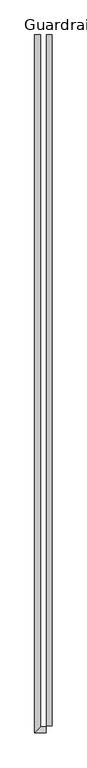
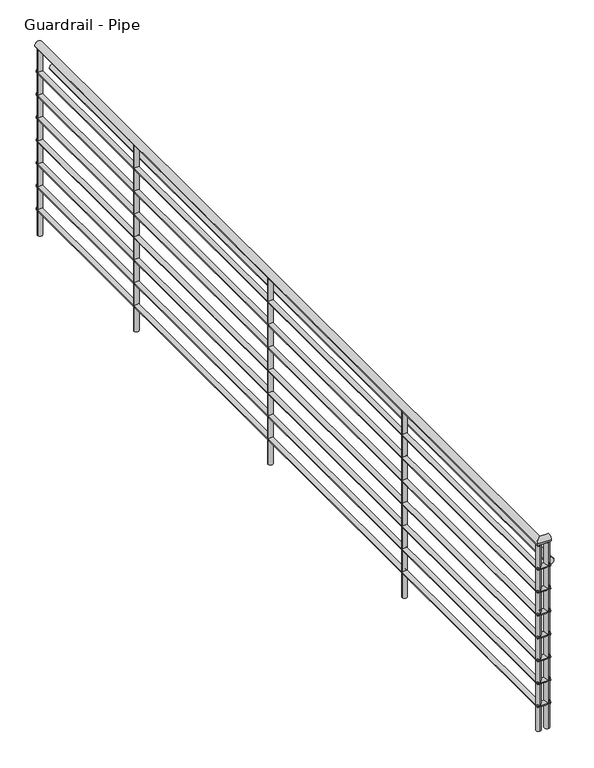
"""IFC4 building model written with IfcOpenShell, lengths in millimetres: railing geometry, Guardrail - Pipe."""

import ifcopenshell
import ifcopenshell.guid

model = None  # the IFC model being written
_history = None  # IfcOwnerHistory: only IFC2X3 demands one
_inside = {}  # id of a spatial element -> (the spatial element, [elements in it])
_under = {}  # id of a project, library or spatial element -> (it, [spatial elements below it])
_declared = {}  # id of a project -> (the project, [libraries it declares])
_typed = {}  # id of a type object -> (the type object, [elements of that type])
_made_of = {}  # id of a material, layer set ... -> (it, [elements and type objects made of it])


def new_model(schema):
    """Start an empty IFC model of exactly this schema.

    Asked for "IFC4X3", IfcOpenShell would pick the latest addendum, in which some entities
    have other attributes; the version numbers below select the first issue.
    IFC2X3 requires an IfcOwnerHistory on every rooted entity: one is made here for all.
    """
    global model, _history
    if schema == "IFC4X3":
        model = ifcopenshell.file(schema_version=(4, 3, 0, 0))
    else:
        model = ifcopenshell.file(schema=schema)
    _inside.clear()
    _under.clear()
    _declared.clear()
    _typed.clear()
    _made_of.clear()
    _history = None
    if model.schema == "IFC2X3":
        org = make("IfcOrganization", Name="unknown")
        user = make(
            "IfcPersonAndOrganization",
            ThePerson=make("IfcPerson", FamilyName="unknown"),
            TheOrganization=org,
        )
        app = make(
            "IfcApplication",
            ApplicationDeveloper=org,
            Version="unknown",
            ApplicationFullName="unknown",
            ApplicationIdentifier="unknown",
        )
        _history = make(
            "IfcOwnerHistory",
            OwningUser=user,
            OwningApplication=app,
            ChangeAction="ADDED",
            CreationDate=0,
        )
    return model


def make(cls, **values):
    """One entity of the class cls with the attributes given. An attribute that is None is left unset."""
    return model.create_entity(
        cls, **{name: value for name, value in values.items() if value is not None}
    )


def rooted(cls, **values):
    """An entity with a GlobalId (a new one), such as an element, a storey or a relation."""
    return make(cls, GlobalId=ifcopenshell.guid.new(), OwnerHistory=_history, **values)


def si_unit(unit_type, name, prefix=None):
    """IfcSIUnit, for example si_unit("LENGTHUNIT", "METRE", prefix="MILLI")."""
    return make("IfcSIUnit", UnitType=unit_type, Prefix=prefix, Name=name)


def assignment(units):
    """IfcUnitAssignment: the units of a project."""
    return None if units is None else make("IfcUnitAssignment", Units=units)


def point(xyz):
    """IfcCartesianPoint."""
    return None if xyz is None else make("IfcCartesianPoint", Coordinates=xyz)


def direction(xyz):
    """IfcDirection."""
    return None if xyz is None else make("IfcDirection", DirectionRatios=xyz)


def frame(location, z_axis=None, x_axis=None):
    """IfcAxis2Placement3D, a coordinate frame: its origin and axes. An axis left out is left unset."""
    return make(
        "IfcAxis2Placement3D",
        Location=point(location),
        Axis=direction(z_axis),
        RefDirection=direction(x_axis),
    )


def frame_2d(location, x_axis=None):
    """IfcAxis2Placement2D, a coordinate frame in the plane: its origin and x axis."""
    return make(
        "IfcAxis2Placement2D", Location=point(location), RefDirection=direction(x_axis)
    )


def origin():
    """The frame at (0, 0, 0) with its axes left unset."""
    return frame((0.0, 0.0, 0.0))


def place(relative_to, where):
    """IfcLocalPlacement: puts the frame where relative to a parent placement (None: the world)."""
    return make(
        "IfcLocalPlacement", PlacementRelTo=relative_to, RelativePlacement=where
    )


def context(
    kind, dimensions, precision=None, world=None, true_north=None, identifier=None
):
    """IfcGeometricRepresentationContext, for example the 3D "Model" context."""
    return make(
        "IfcGeometricRepresentationContext",
        ContextIdentifier=identifier,
        ContextType=kind,
        CoordinateSpaceDimension=dimensions,
        Precision=precision,
        WorldCoordinateSystem=world,
        TrueNorth=true_north,
    )


def project(units=None, contexts=None):
    """IfcProject with its units and contexts."""
    return rooted(
        "IfcProject",
        Name="project",
        RepresentationContexts=contexts,
        UnitsInContext=assignment(units),
    )


def spatial(cls, under=None, at=None, **own):
    """A site, building, storey or space (cls), placed at a placement, below another one or the project."""
    s = rooted(cls, ObjectPlacement=at, **own)
    if under is not None:
        _under.setdefault(under.id(), (under, []))[1].append(s)
    return s


def circle_curve(where, radius):
    """IfcCircle in the frame where."""
    return make("IfcCircle", Position=where, Radius=radius)


def ellipse_curve(where, semi_axis1, semi_axis2):
    """IfcEllipse in the frame where."""
    return make(
        "IfcEllipse", Position=where, SemiAxis1=semi_axis1, SemiAxis2=semi_axis2
    )


def trimmed(basis, trim1, trim2, sense, master):
    """IfcTrimmedCurve: the piece of a basis curve between two trims."""
    return make(
        "IfcTrimmedCurve",
        BasisCurve=basis,
        Trim1=trim1,
        Trim2=trim2,
        SenseAgreement=sense,
        MasterRepresentation=master,
    )


def segment(curve, same_sense, transition):
    """IfcCompositeCurveSegment."""
    return make(
        "IfcCompositeCurveSegment",
        Transition=transition,
        SameSense=same_sense,
        ParentCurve=curve,
    )


def composite_curve(segments, self_intersect=None):
    """IfcCompositeCurve: segments joined end to end."""
    return make("IfcCompositeCurve", Segments=segments, SelfIntersect=self_intersect)


def outline(outer, holes=None, kind="AREA"):
    """IfcArbitraryClosedProfileDef: a profile drawn as a closed curve; with holes, ...WithVoids."""
    if holes is None:
        return make("IfcArbitraryClosedProfileDef", ProfileType=kind, OuterCurve=outer)
    return make(
        "IfcArbitraryProfileDefWithVoids",
        ProfileType=kind,
        OuterCurve=outer,
        InnerCurves=holes,
    )


def extrude(swept, where, along, depth):
    """IfcExtrudedAreaSolid: the profile swept, set in the frame where, extruded along a direction by depth."""
    return make(
        "IfcExtrudedAreaSolid",
        SweptArea=swept,
        Position=where,
        ExtrudedDirection=direction(along),
        Depth=depth,
    )


def shape(context_of_items, identifier, shape_type, items):
    """IfcShapeRepresentation: the items that make up one representation, for example the "Body"."""
    return make(
        "IfcShapeRepresentation",
        ContextOfItems=context_of_items,
        RepresentationIdentifier=identifier,
        RepresentationType=shape_type,
        Items=items,
    )


def source(mapping_origin, context_of_items, identifier, shape_type, items):
    """IfcRepresentationMap: a shape defined once, which mapped items show again and again."""
    return make(
        "IfcRepresentationMap",
        MappingOrigin=mapping_origin,
        MappedRepresentation=shape(context_of_items, identifier, shape_type, items),
    )


def transform(
    local_origin,
    x_axis=None,
    y_axis=None,
    z_axis=None,
    scale=None,
    scale2=None,
    scale3=None,
    uniform=True,
):
    """IfcCartesianTransformationOperator3D, or its non-uniform kind. x_axis, y_axis, z_axis: its Axis1, 2, 3."""
    if uniform:
        return make(
            "IfcCartesianTransformationOperator3D",
            Axis1=direction(x_axis),
            Axis2=direction(y_axis),
            LocalOrigin=point(local_origin),
            Scale=scale,
            Axis3=direction(z_axis),
        )
    return make(
        "IfcCartesianTransformationOperator3DnonUniform",
        Axis1=direction(x_axis),
        Axis2=direction(y_axis),
        LocalOrigin=point(local_origin),
        Scale=scale,
        Axis3=direction(z_axis),
        Scale2=scale2,
        Scale3=scale3,
    )


def mapped(mapping_source, mapping_target):
    """IfcMappedItem: shows the shape of a source again, moved by a transform."""
    return make(
        "IfcMappedItem", MappingSource=mapping_source, MappingTarget=mapping_target
    )


def made_of(thing, what):
    """Note that an element or type object is made of a material, layer set ...; save() writes the relation."""
    if what is not None:
        _made_of.setdefault(what.id(), (what, []))[1].append(thing)
    return thing


def element(
    cls,
    number,
    at=None,
    inside=None,
    cuts=None,
    type_object=None,
    material=None,
    context=None,
    identifier="Body",
    shape_type=None,
    held_by="IfcProductDefinitionShape",
    body=None,
    shapes=None,
    **own,
):
    """One element of the class cls, such as IfcWall. Its Tag is "e" and its number.

    at: its placement. inside: the storey or other place that contains it. cuts: it is an
    opening in that element (IfcRelVoidsElement). A single representation is given by context,
    identifier, shape_type and body (its items); several are given by shapes. held_by: the class
    of the entity that holds the representations. save() writes the other relations.
    """
    e = rooted(cls, Tag="e%d" % number, ObjectPlacement=at, **own)
    if body is not None:
        shapes = [shape(context, identifier, shape_type, body)]
    if shapes is not None:
        e.Representation = make(held_by, Representations=shapes)
    if inside is not None:
        _inside.setdefault(inside.id(), (inside, []))[1].append(e)
    if cuts is not None:
        rooted(
            "IfcRelVoidsElement", RelatingBuildingElement=cuts, RelatedOpeningElement=e
        )
    if type_object is not None:
        _typed.setdefault(type_object.id(), (type_object, []))[1].append(e)
    return made_of(e, material)


def aggregate(whole, parts):
    """IfcRelAggregates: a whole, such as a stair, and the parts it consists of."""
    return rooted("IfcRelAggregates", RelatingObject=whole, RelatedObjects=parts)


def save(model, path):
    """Write the relations noted so far, then the file.

    IfcRelAggregates (storeys below a building ...), IfcRelContainedInSpatialStructure (elements
    in a storey), IfcRelDefinesByType, IfcRelAssociatesMaterial and IfcRelDeclares: one each for
    every whole, place, type object, material and project.
    """
    for whole, parts in _under.values():
        aggregate(whole, parts)
    for where, things in _inside.values():
        rooted(
            "IfcRelContainedInSpatialStructure",
            RelatedElements=things,
            RelatingStructure=where,
        )
    for kind, things in _typed.values():
        rooted("IfcRelDefinesByType", RelatedObjects=things, RelatingType=kind)
    for what, things in _made_of.values():
        rooted("IfcRelAssociatesMaterial", RelatedObjects=things, RelatingMaterial=what)
    for by, libraries in _declared.values():
        rooted("IfcRelDeclares", RelatingContext=by, RelatedDefinitions=libraries)
    model.write(path)


def plane_surface(at):
    """IfcPlane: the flat surface through the origin of the frame at, square to its z axis."""
    return make("IfcPlane", Position=at)


def cylinder_surface(at, radius):
    """IfcCylindricalSurface: all points at the distance radius from the z axis of the frame at."""
    return make("IfcCylindricalSurface", Position=at, Radius=radius)


def advanced_brep(points, edges, surfaces, faces):
    """IfcAdvancedBrep: a solid bounded by faces that lie on surfaces and meet in shared edges.

    An edge is (start, end): straight between two places in points (the first is 0);
    or (start, end, curve); or (start, end, curve, False) where it runs against its curve.
    A face is (place in surfaces, loops), or (place, loops, False) where it looks against
    its surface's normal. A loop lists edges by number (the first is 1), with a minus sign
    where the edge is run from its end to its start. The first loop is the outer one.
    """
    corners = [point(p) for p in points]
    vertices = [make("IfcVertexPoint", VertexGeometry=c) for c in corners]
    made = []
    for start, end, *more in edges:
        made.append(
            make(
                "IfcEdgeCurve",
                EdgeStart=vertices[start],
                EdgeEnd=vertices[end],
                EdgeGeometry=more[0] if more else make("IfcPolyline", Points=[corners[start], corners[end]]),
                SameSense=more[1] if len(more) > 1 else True,
            )
        )
    hull = []
    for where, loops, *sense in faces:
        bounds = []
        for j, loop in enumerate(loops):
            ring = [make("IfcOrientedEdge", EdgeElement=made[abs(k) - 1], Orientation=k > 0) for k in loop]
            bounds.append(
                make(
                    "IfcFaceOuterBound" if j == 0 else "IfcFaceBound",
                    Bound=make("IfcEdgeLoop", EdgeList=ring),
                    Orientation=True,
                )
            )
        hull.append(make("IfcAdvancedFace", Bounds=bounds, FaceSurface=surfaces[where], SameSense=sense[0] if sense else True))
    return make("IfcAdvancedBrep", Outer=make("IfcClosedShell", CfsFaces=hull))


def guardrail_pipe_4d6737b3(model_context):
    return source(origin(), model_context, "Body", "SolidModel", [
        advanced_brep(
        [(-10682.1293787, 596.0663228, 4705.35), (-10720.2293787, 596.0663228, 4705.35), (-10682.1293787, -3931.4836772, 4705.35), (-10720.2293787, -3969.5836772, 4705.35), (-10645.1029016, -3931.4836772, 4705.35), (-10645.1029016, -3969.5836772, 4705.35)],
        [
            (0, 1, circle_curve(frame((-10701.1793787, 596.0663228, 4705.35), z_axis=(0.0, 1.0, 0.0), x_axis=(-1.0, 0.0, 0.0)), 19.05)),
            (1, 0, circle_curve(frame((-10701.1793787, 596.0663228, 4705.35), z_axis=(0.0, 1.0, 0.0), x_axis=(-1.0, 0.0, 0.0)), 19.05)),
            (2, 3, ellipse_curve(frame((-10701.1793787, -3950.5336772, 4705.35), z_axis=(-0.7071067811865456, 0.7071067811865493, 0.0), x_axis=(-0.7071067811865492, -0.7071067811865458, 0.0)), 26.9407684, 19.05)),
            (3, 1),
            (0, 2),
            (3, 2, ellipse_curve(frame((-10701.1793787, -3950.5336772, 4705.35), z_axis=(-0.7071067811865456, 0.7071067811865493, 0.0), x_axis=(-0.7071067811865492, -0.7071067811865458, 0.0)), 26.9407684, 19.05)),
            (4, 5, circle_curve(frame((-10645.1029016, -3950.5336772, 4705.35), z_axis=(1.0, 0.0, 0.0), x_axis=(0.0, -1.0, 0.0)), 19.05)),
            (5, 4, circle_curve(frame((-10645.1029016, -3950.5336772, 4705.35), z_axis=(1.0, 0.0, 0.0), x_axis=(0.0, -1.0, 0.0)), 19.05)),
            (5, 3),
            (2, 4),
        ],
        [
            plane_surface(frame((-10701.1793787, 596.0663228, 4724.4), z_axis=(0.0, 1.0, 0.0), x_axis=(0.0, 0.0, 1.0))),
            cylinder_surface(frame((-10701.1793787, -3950.5336772, 4705.35), z_axis=(0.0, -1.0, 0.0), x_axis=(-1.0, 0.0, 0.0)), 19.05),
            plane_surface(frame((-10645.1029016, -3950.5336772, 4724.4), z_axis=(1.0, 0.0, 0.0), x_axis=(0.0, -1.0, 0.0))),
            cylinder_surface(frame((-10645.1029016, -3950.5336772, 4705.35), z_axis=(1.0, 0.0, 0.0), x_axis=(0.0, -1.0, 0.0)), 19.05),
        ],
        [
            (0, [[1, 2]]),
            (1, [[3, 4, -1, 5]]),
            (1, [[6, -5, -2, -4]]),
            (2, [[7, 8]]),
            (3, [[-8, 9, -3, 10]]),
            (3, [[-7, -10, -6, -9]]),
        ],
    ),
        advanced_brep(
        [(-10688.4793787, 596.0663228, 4559.3), (-10713.8793787, 596.0663228, 4559.3), (-10688.4793787, -3937.8336772, 4559.3), (-10713.8793787, -3963.2336772, 4559.3), (-10645.1029016, -3937.8336772, 4559.3), (-10645.1029016, -3963.2336772, 4559.3)],
        [
            (0, 1, circle_curve(frame((-10701.1793787, 596.0663228, 4559.3), z_axis=(0.0, 1.0, 0.0), x_axis=(-1.0, 0.0, 0.0)), 12.7)),
            (1, 0, circle_curve(frame((-10701.1793787, 596.0663228, 4559.3), z_axis=(0.0, 1.0, 0.0), x_axis=(-1.0, 0.0, 0.0)), 12.7)),
            (2, 3, ellipse_curve(frame((-10701.1793787, -3950.5336772, 4559.3), z_axis=(-0.7071067811865456, 0.7071067811865493, 0.0), x_axis=(-0.7071067811865492, -0.7071067811865458, 0.0)), 17.9605122, 12.7)),
            (3, 1),
            (0, 2),
            (3, 2, ellipse_curve(frame((-10701.1793787, -3950.5336772, 4559.3), z_axis=(-0.7071067811865456, 0.7071067811865493, 0.0), x_axis=(-0.7071067811865492, -0.7071067811865458, 0.0)), 17.9605122, 12.7)),
            (4, 5, circle_curve(frame((-10645.1029016, -3950.5336772, 4559.3), z_axis=(1.0, 0.0, 0.0), x_axis=(0.0, -1.0, 0.0)), 12.7)),
            (5, 4, circle_curve(frame((-10645.1029016, -3950.5336772, 4559.3), z_axis=(1.0, 0.0, 0.0), x_axis=(0.0, -1.0, 0.0)), 12.7)),
            (4, 2),
            (3, 5),
        ],
        [
            plane_surface(frame((-10701.1793787, 596.0663228, 4572.0), z_axis=(0.0, 1.0, 0.0), x_axis=(0.0, 0.0, 1.0))),
            cylinder_surface(frame((-10701.1793787, -3950.5336772, 4559.3), z_axis=(0.0, -1.0, 0.0), x_axis=(-1.0, 0.0, 0.0)), 12.7),
            plane_surface(frame((-10645.1029016, -3950.5336772, 4572.0), z_axis=(1.0, 0.0, 0.0), x_axis=(0.0, -1.0, 0.0))),
            cylinder_surface(frame((-10645.1029016, -3950.5336772, 4559.3), z_axis=(1.0, 0.0, 0.0), x_axis=(0.0, -1.0, 0.0)), 12.7),
        ],
        [
            (0, [[1, 2]]),
            (1, [[3, 4, -1, 5]]),
            (1, [[6, -5, -2, -4]]),
            (2, [[7, 8]]),
            (3, [[-7, 9, -6, 10]]),
            (3, [[-8, -10, -3, -9]]),
        ],
    ),
        advanced_brep(
        [(-10605.9293787, -3925.1336772, 4552.95), (-10644.0293787, -3925.1336772, 4552.95), (-10605.9293787, 596.0663228, 4552.95), (-10644.0293787, 596.0663228, 4552.95)],
        [
            (0, 1, circle_curve(frame((-10624.9793787, -3925.1336772, 4552.95), z_axis=(0.0, -1.0, 0.0), x_axis=(-1.0, 0.0, 0.0)), 19.05)),
            (1, 0, circle_curve(frame((-10624.9793787, -3925.1336772, 4552.95), z_axis=(0.0, -1.0, 0.0), x_axis=(-1.0, 0.0, 0.0)), 19.05)),
            (2, 3, circle_curve(frame((-10624.9793787, 596.0663228, 4552.95), z_axis=(0.0, 1.0, 0.0), x_axis=(-1.0, 0.0, 0.0)), 19.05)),
            (3, 2, circle_curve(frame((-10624.9793787, 596.0663228, 4552.95), z_axis=(0.0, 1.0, 0.0), x_axis=(-1.0, 0.0, 0.0)), 19.05)),
            (1, 3),
            (2, 0),
        ],
        [
            plane_surface(frame((-10624.9793787, -3925.1336772, 4572.0), z_axis=(0.0, -1.0, 0.0), x_axis=(0.0, 0.0, 1.0))),
            plane_surface(frame((-10624.9793787, 596.0663228, 4572.0), z_axis=(0.0, 1.0, 0.0), x_axis=(0.0, 0.0, 1.0))),
            cylinder_surface(frame((-10624.9793787, -3925.1336772, 4552.95), z_axis=(0.0, -1.0, 0.0), x_axis=(-1.0, 0.0, 0.0)), 19.05),
        ],
        [
            (0, [[1, 2]]),
            (1, [[3, 4]]),
            (2, [[-2, 5, -3, 6]]),
            (2, [[-1, -6, -4, -5]]),
        ],
    ),
        advanced_brep(
        [(-10688.4793787, 596.0663228, 4432.3), (-10713.8793787, 596.0663228, 4432.3), (-10688.4793787, -3937.8336772, 4432.3), (-10713.8793787, -3963.2336772, 4432.3), (-10645.1029016, -3937.8336772, 4432.3), (-10645.1029016, -3963.2336772, 4432.3)],
        [
            (0, 1, circle_curve(frame((-10701.1793787, 596.0663228, 4432.3), z_axis=(0.0, 1.0, 0.0), x_axis=(-1.0, 0.0, 0.0)), 12.7)),
            (1, 0, circle_curve(frame((-10701.1793787, 596.0663228, 4432.3), z_axis=(0.0, 1.0, 0.0), x_axis=(-1.0, 0.0, 0.0)), 12.7)),
            (2, 3, ellipse_curve(frame((-10701.1793787, -3950.5336772, 4432.3), z_axis=(-0.7071067811865456, 0.7071067811865493, 0.0), x_axis=(-0.7071067811865492, -0.7071067811865458, 0.0)), 17.9605122, 12.7)),
            (3, 1),
            (0, 2),
            (3, 2, ellipse_curve(frame((-10701.1793787, -3950.5336772, 4432.3), z_axis=(-0.7071067811865456, 0.7071067811865493, 0.0), x_axis=(-0.7071067811865492, -0.7071067811865458, 0.0)), 17.9605122, 12.7)),
            (4, 5, circle_curve(frame((-10645.1029016, -3950.5336772, 4432.3), z_axis=(1.0, 0.0, 0.0), x_axis=(0.0, -1.0, 0.0)), 12.7)),
            (5, 4, circle_curve(frame((-10645.1029016, -3950.5336772, 4432.3), z_axis=(1.0, 0.0, 0.0), x_axis=(0.0, -1.0, 0.0)), 12.7)),
            (4, 2),
            (3, 5),
        ],
        [
            plane_surface(frame((-10701.1793787, 596.0663228, 4445.0), z_axis=(0.0, 1.0, 0.0), x_axis=(0.0, 0.0, 1.0))),
            cylinder_surface(frame((-10701.1793787, -3950.5336772, 4432.3), z_axis=(0.0, -1.0, 0.0), x_axis=(-1.0, 0.0, 0.0)), 12.7),
            plane_surface(frame((-10645.1029016, -3950.5336772, 4445.0), z_axis=(1.0, 0.0, 0.0), x_axis=(0.0, -1.0, 0.0))),
            cylinder_surface(frame((-10645.1029016, -3950.5336772, 4432.3), z_axis=(1.0, 0.0, 0.0), x_axis=(0.0, -1.0, 0.0)), 12.7),
        ],
        [
            (0, [[1, 2]]),
            (1, [[3, 4, -1, 5]]),
            (1, [[6, -5, -2, -4]]),
            (2, [[7, 8]]),
            (3, [[-7, 9, -6, 10]]),
            (3, [[-8, -10, -3, -9]]),
        ],
    ),
        advanced_brep(
        [(-10688.4793787, 596.0663228, 4305.3), (-10713.8793787, 596.0663228, 4305.3), (-10688.4793787, -3937.8336772, 4305.3), (-10713.8793787, -3963.2336772, 4305.3), (-10645.1029016, -3937.8336772, 4305.3), (-10645.1029016, -3963.2336772, 4305.3)],
        [
            (0, 1, circle_curve(frame((-10701.1793787, 596.0663228, 4305.3), z_axis=(0.0, 1.0, 0.0), x_axis=(-1.0, 0.0, 0.0)), 12.7)),
            (1, 0, circle_curve(frame((-10701.1793787, 596.0663228, 4305.3), z_axis=(0.0, 1.0, 0.0), x_axis=(-1.0, 0.0, 0.0)), 12.7)),
            (2, 3, ellipse_curve(frame((-10701.1793787, -3950.5336772, 4305.3), z_axis=(-0.7071067811865456, 0.7071067811865493, 0.0), x_axis=(-0.7071067811865492, -0.7071067811865458, 0.0)), 17.9605122, 12.7)),
            (3, 1),
            (0, 2),
            (3, 2, ellipse_curve(frame((-10701.1793787, -3950.5336772, 4305.3), z_axis=(-0.7071067811865456, 0.7071067811865493, 0.0), x_axis=(-0.7071067811865492, -0.7071067811865458, 0.0)), 17.9605122, 12.7)),
            (4, 5, circle_curve(frame((-10645.1029016, -3950.5336772, 4305.3), z_axis=(1.0, 0.0, 0.0), x_axis=(0.0, -1.0, 0.0)), 12.7)),
            (5, 4, circle_curve(frame((-10645.1029016, -3950.5336772, 4305.3), z_axis=(1.0, 0.0, 0.0), x_axis=(0.0, -1.0, 0.0)), 12.7)),
            (4, 2),
            (3, 5),
        ],
        [
            plane_surface(frame((-10701.1793787, 596.0663228, 4318.0), z_axis=(0.0, 1.0, 0.0), x_axis=(0.0, 0.0, 1.0))),
            cylinder_surface(frame((-10701.1793787, -3950.5336772, 4305.3), z_axis=(0.0, -1.0, 0.0), x_axis=(-1.0, 0.0, 0.0)), 12.7),
            plane_surface(frame((-10645.1029016, -3950.5336772, 4318.0), z_axis=(1.0, 0.0, 0.0), x_axis=(0.0, -1.0, 0.0))),
            cylinder_surface(frame((-10645.1029016, -3950.5336772, 4305.3), z_axis=(1.0, 0.0, 0.0), x_axis=(0.0, -1.0, 0.0)), 12.7),
        ],
        [
            (0, [[1, 2]]),
            (1, [[3, 4, -1, 5]]),
            (1, [[6, -5, -2, -4]]),
            (2, [[7, 8]]),
            (3, [[-7, 9, -6, 10]]),
            (3, [[-8, -10, -3, -9]]),
        ],
    ),
        advanced_brep(
        [(-10688.4793787, 596.0663228, 4178.3), (-10713.8793787, 596.0663228, 4178.3), (-10688.4793787, -3937.8336772, 4178.3), (-10713.8793787, -3963.2336772, 4178.3), (-10645.1029016, -3937.8336772, 4178.3), (-10645.1029016, -3963.2336772, 4178.3)],
        [
            (0, 1, circle_curve(frame((-10701.1793787, 596.0663228, 4178.3), z_axis=(0.0, 1.0, 0.0), x_axis=(-1.0, 0.0, 0.0)), 12.7)),
            (1, 0, circle_curve(frame((-10701.1793787, 596.0663228, 4178.3), z_axis=(0.0, 1.0, 0.0), x_axis=(-1.0, 0.0, 0.0)), 12.7)),
            (2, 3, ellipse_curve(frame((-10701.1793787, -3950.5336772, 4178.3), z_axis=(-0.7071067811865456, 0.7071067811865493, 0.0), x_axis=(-0.7071067811865492, -0.7071067811865458, 0.0)), 17.9605122, 12.7)),
            (3, 1),
            (0, 2),
            (3, 2, ellipse_curve(frame((-10701.1793787, -3950.5336772, 4178.3), z_axis=(-0.7071067811865456, 0.7071067811865493, 0.0), x_axis=(-0.7071067811865492, -0.7071067811865458, 0.0)), 17.9605122, 12.7)),
            (4, 5, circle_curve(frame((-10645.1029016, -3950.5336772, 4178.3), z_axis=(1.0, 0.0, 0.0), x_axis=(0.0, -1.0, 0.0)), 12.7)),
            (5, 4, circle_curve(frame((-10645.1029016, -3950.5336772, 4178.3), z_axis=(1.0, 0.0, 0.0), x_axis=(0.0, -1.0, 0.0)), 12.7)),
            (4, 2),
            (3, 5),
        ],
        [
            plane_surface(frame((-10701.1793787, 596.0663228, 4191.0), z_axis=(0.0, 1.0, 0.0), x_axis=(0.0, 0.0, 1.0))),
            cylinder_surface(frame((-10701.1793787, -3950.5336772, 4178.3), z_axis=(0.0, -1.0, 0.0), x_axis=(-1.0, 0.0, 0.0)), 12.7),
            plane_surface(frame((-10645.1029016, -3950.5336772, 4191.0), z_axis=(1.0, 0.0, 0.0), x_axis=(0.0, -1.0, 0.0))),
            cylinder_surface(frame((-10645.1029016, -3950.5336772, 4178.3), z_axis=(1.0, 0.0, 0.0), x_axis=(0.0, -1.0, 0.0)), 12.7),
        ],
        [
            (0, [[1, 2]]),
            (1, [[3, 4, -1, 5]]),
            (1, [[6, -5, -2, -4]]),
            (2, [[7, 8]]),
            (3, [[-7, 9, -6, 10]]),
            (3, [[-8, -10, -3, -9]]),
        ],
    ),
        advanced_brep(
        [(-10688.4793787, 596.0663228, 4051.3), (-10713.8793787, 596.0663228, 4051.3), (-10688.4793787, -3937.8336772, 4051.3), (-10713.8793787, -3963.2336772, 4051.3), (-10645.1029016, -3937.8336772, 4051.3), (-10645.1029016, -3963.2336772, 4051.3)],
        [
            (0, 1, circle_curve(frame((-10701.1793787, 596.0663228, 4051.3), z_axis=(0.0, 1.0, 0.0), x_axis=(-1.0, 0.0, 0.0)), 12.7)),
            (1, 0, circle_curve(frame((-10701.1793787, 596.0663228, 4051.3), z_axis=(0.0, 1.0, 0.0), x_axis=(-1.0, 0.0, 0.0)), 12.7)),
            (2, 3, ellipse_curve(frame((-10701.1793787, -3950.5336772, 4051.3), z_axis=(-0.7071067811865456, 0.7071067811865493, 0.0), x_axis=(-0.7071067811865492, -0.7071067811865458, 0.0)), 17.9605122, 12.7)),
            (3, 1),
            (0, 2),
            (3, 2, ellipse_curve(frame((-10701.1793787, -3950.5336772, 4051.3), z_axis=(-0.7071067811865456, 0.7071067811865493, 0.0), x_axis=(-0.7071067811865492, -0.7071067811865458, 0.0)), 17.9605122, 12.7)),
            (4, 5, circle_curve(frame((-10645.1029016, -3950.5336772, 4051.3), z_axis=(1.0, 0.0, 0.0), x_axis=(0.0, -1.0, 0.0)), 12.7)),
            (5, 4, circle_curve(frame((-10645.1029016, -3950.5336772, 4051.3), z_axis=(1.0, 0.0, 0.0), x_axis=(0.0, -1.0, 0.0)), 12.7)),
            (4, 2),
            (3, 5),
        ],
        [
            plane_surface(frame((-10701.1793787, 596.0663228, 4064.0), z_axis=(0.0, 1.0, 0.0), x_axis=(0.0, 0.0, 1.0))),
            cylinder_surface(frame((-10701.1793787, -3950.5336772, 4051.3), z_axis=(0.0, -1.0, 0.0), x_axis=(-1.0, 0.0, 0.0)), 12.7),
            plane_surface(frame((-10645.1029016, -3950.5336772, 4064.0), z_axis=(1.0, 0.0, 0.0), x_axis=(0.0, -1.0, 0.0))),
            cylinder_surface(frame((-10645.1029016, -3950.5336772, 4051.3), z_axis=(1.0, 0.0, 0.0), x_axis=(0.0, -1.0, 0.0)), 12.7),
        ],
        [
            (0, [[1, 2]]),
            (1, [[3, 4, -1, 5]]),
            (1, [[6, -5, -2, -4]]),
            (2, [[7, 8]]),
            (3, [[-7, 9, -6, 10]]),
            (3, [[-8, -10, -3, -9]]),
        ],
    ),
        advanced_brep(
        [(-10688.4793787, 596.0663228, 3924.3), (-10713.8793787, 596.0663228, 3924.3), (-10688.4793787, -3937.8336772, 3924.3), (-10713.8793787, -3963.2336772, 3924.3), (-10645.1029016, -3937.8336772, 3924.3), (-10645.1029016, -3963.2336772, 3924.3)],
        [
            (0, 1, circle_curve(frame((-10701.1793787, 596.0663228, 3924.3), z_axis=(0.0, 1.0, 0.0), x_axis=(-1.0, 0.0, 0.0)), 12.7)),
            (1, 0, circle_curve(frame((-10701.1793787, 596.0663228, 3924.3), z_axis=(0.0, 1.0, 0.0), x_axis=(-1.0, 0.0, 0.0)), 12.7)),
            (2, 3, ellipse_curve(frame((-10701.1793787, -3950.5336772, 3924.3), z_axis=(-0.7071067811865456, 0.7071067811865493, 0.0), x_axis=(-0.7071067811865492, -0.7071067811865458, 0.0)), 17.9605122, 12.7)),
            (3, 1),
            (0, 2),
            (3, 2, ellipse_curve(frame((-10701.1793787, -3950.5336772, 3924.3), z_axis=(-0.7071067811865456, 0.7071067811865493, 0.0), x_axis=(-0.7071067811865492, -0.7071067811865458, 0.0)), 17.9605122, 12.7)),
            (4, 5, circle_curve(frame((-10645.1029016, -3950.5336772, 3924.3), z_axis=(1.0, 0.0, 0.0), x_axis=(0.0, -1.0, 0.0)), 12.7)),
            (5, 4, circle_curve(frame((-10645.1029016, -3950.5336772, 3924.3), z_axis=(1.0, 0.0, 0.0), x_axis=(0.0, -1.0, 0.0)), 12.7)),
            (4, 2),
            (3, 5),
        ],
        [
            plane_surface(frame((-10701.1793787, 596.0663228, 3937.0), z_axis=(0.0, 1.0, 0.0), x_axis=(0.0, 0.0, 1.0))),
            cylinder_surface(frame((-10701.1793787, -3950.5336772, 3924.3), z_axis=(0.0, -1.0, 0.0), x_axis=(-1.0, 0.0, 0.0)), 12.7),
            plane_surface(frame((-10645.1029016, -3950.5336772, 3937.0), z_axis=(1.0, 0.0, 0.0), x_axis=(0.0, -1.0, 0.0))),
            cylinder_surface(frame((-10645.1029016, -3950.5336772, 3924.3), z_axis=(1.0, 0.0, 0.0), x_axis=(0.0, -1.0, 0.0)), 12.7),
        ],
        [
            (0, [[1, 2]]),
            (1, [[3, 4, -1, 5]]),
            (1, [[6, -5, -2, -4]]),
            (2, [[7, 8]]),
            (3, [[-7, 9, -6, 10]]),
            (3, [[-8, -10, -3, -9]]),
        ],
    ),
        advanced_brep(
        [(-10688.4793787, 596.0663228, 3797.3), (-10713.8793787, 596.0663228, 3797.3), (-10688.4793787, -3937.8336772, 3797.3), (-10713.8793787, -3963.2336772, 3797.3), (-10645.1029016, -3937.8336772, 3797.3), (-10645.1029016, -3963.2336772, 3797.3)],
        [
            (0, 1, circle_curve(frame((-10701.1793787, 596.0663228, 3797.3), z_axis=(0.0, 1.0, 0.0), x_axis=(-1.0, 0.0, 0.0)), 12.7)),
            (1, 0, circle_curve(frame((-10701.1793787, 596.0663228, 3797.3), z_axis=(0.0, 1.0, 0.0), x_axis=(-1.0, 0.0, 0.0)), 12.7)),
            (2, 3, ellipse_curve(frame((-10701.1793787, -3950.5336772, 3797.3), z_axis=(-0.7071067811865456, 0.7071067811865493, 0.0), x_axis=(-0.7071067811865492, -0.7071067811865458, 0.0)), 17.9605122, 12.7)),
            (3, 1),
            (0, 2),
            (3, 2, ellipse_curve(frame((-10701.1793787, -3950.5336772, 3797.3), z_axis=(-0.7071067811865456, 0.7071067811865493, 0.0), x_axis=(-0.7071067811865492, -0.7071067811865458, 0.0)), 17.9605122, 12.7)),
            (4, 5, circle_curve(frame((-10645.1029016, -3950.5336772, 3797.3), z_axis=(1.0, 0.0, 0.0), x_axis=(0.0, -1.0, 0.0)), 12.7)),
            (5, 4, circle_curve(frame((-10645.1029016, -3950.5336772, 3797.3), z_axis=(1.0, 0.0, 0.0), x_axis=(0.0, -1.0, 0.0)), 12.7)),
            (4, 2),
            (3, 5),
        ],
        [
            plane_surface(frame((-10701.1793787, 596.0663228, 3810.0), z_axis=(0.0, 1.0, 0.0), x_axis=(0.0, 0.0, 1.0))),
            cylinder_surface(frame((-10701.1793787, -3950.5336772, 3797.3), z_axis=(0.0, -1.0, 0.0), x_axis=(-1.0, 0.0, 0.0)), 12.7),
            plane_surface(frame((-10645.1029016, -3950.5336772, 3810.0), z_axis=(1.0, 0.0, 0.0), x_axis=(0.0, -1.0, 0.0))),
            cylinder_surface(frame((-10645.1029016, -3950.5336772, 3797.3), z_axis=(1.0, 0.0, 0.0), x_axis=(0.0, -1.0, 0.0)), 12.7),
        ],
        [
            (0, [[1, 2]]),
            (1, [[3, 4, -1, 5]]),
            (1, [[6, -5, -2, -4]]),
            (2, [[7, 8]]),
            (3, [[-7, 9, -6, 10]]),
            (3, [[-8, -10, -3, -9]]),
        ],
    ),
        extrude(outline(composite_curve([segment(trimmed(circle_curve(frame_2d((-10701.1793787, -292.9336772)), 12.7), [point((-10688.4793787, -292.9336772))], [point((-10713.8793787, -292.9336772))], False, "CARTESIAN"), True, "CONTINUOUS"), segment(trimmed(circle_curve(frame_2d((-10701.1793787, -292.9336772)), 12.7), [point((-10713.8793787, -292.9336772))], [point((-10688.4793787, -292.9336772))], False, "CARTESIAN"), True, "CONTINUOUS")], self_intersect=False)), frame((0.0, 0.0, 3657.6), z_axis=(0.0, 0.0, 1.0), x_axis=(1.0, 0.0, 0.0)), (0.0, 0.0, 1.0), 1028.7),
        extrude(outline(composite_curve([segment(trimmed(circle_curve(frame_2d((-10701.1793787, -1512.1336772)), 12.7), [point((-10688.4793787, -1512.1336772))], [point((-10713.8793787, -1512.1336772))], False, "CARTESIAN"), True, "CONTINUOUS"), segment(trimmed(circle_curve(frame_2d((-10701.1793787, -1512.1336772)), 12.7), [point((-10713.8793787, -1512.1336772))], [point((-10688.4793787, -1512.1336772))], False, "CARTESIAN"), True, "CONTINUOUS")], self_intersect=False)), frame((0.0, 0.0, 3657.6), z_axis=(0.0, 0.0, 1.0), x_axis=(1.0, 0.0, 0.0)), (0.0, 0.0, 1.0), 1028.7),
        extrude(outline(composite_curve([segment(trimmed(circle_curve(frame_2d((-10701.1793787, -2731.3336772)), 12.7), [point((-10688.4793787, -2731.3336772))], [point((-10713.8793787, -2731.3336772))], False, "CARTESIAN"), True, "CONTINUOUS"), segment(trimmed(circle_curve(frame_2d((-10701.1793787, -2731.3336772)), 12.7), [point((-10713.8793787, -2731.3336772))], [point((-10688.4793787, -2731.3336772))], False, "CARTESIAN"), True, "CONTINUOUS")], self_intersect=False)), frame((0.0, 0.0, 3657.6), z_axis=(0.0, 0.0, 1.0), x_axis=(1.0, 0.0, 0.0)), (0.0, 0.0, 1.0), 1028.7),
        extrude(outline(composite_curve([segment(trimmed(circle_curve(frame_2d((-10701.1793787, -3950.5336772)), 12.7), [point((-10701.1793787, -3937.8336772))], [point((-10701.1793787, -3963.2336772))], False, "CARTESIAN"), True, "CONTINUOUS"), segment(trimmed(circle_curve(frame_2d((-10701.1793787, -3950.5336772)), 12.7), [point((-10701.1793787, -3963.2336772))], [point((-10701.1793787, -3937.8336772))], False, "CARTESIAN"), True, "CONTINUOUS")], self_intersect=False)), frame((0.0, 0.0, 3657.6), z_axis=(0.0, 0.0, 1.0), x_axis=(1.0, 0.0, 0.0)), (0.0, 0.0, 1.0), 1028.7),
        extrude(outline(composite_curve([segment(trimmed(circle_curve(frame_2d((-10701.1793787, 583.3663228)), 12.7), [point((-10688.4793787, 583.3663228))], [point((-10713.8793787, 583.3663228))], False, "CARTESIAN"), True, "CONTINUOUS"), segment(trimmed(circle_curve(frame_2d((-10701.1793787, 583.3663228)), 12.7), [point((-10713.8793787, 583.3663228))], [point((-10688.4793787, 583.3663228))], False, "CARTESIAN"), True, "CONTINUOUS")], self_intersect=False)), frame((0.0, 0.0, 3657.6), z_axis=(0.0, 0.0, 1.0), x_axis=(1.0, 0.0, 0.0)), (0.0, 0.0, 1.0), 1028.7),
        extrude(outline(composite_curve([segment(trimmed(circle_curve(frame_2d((-10657.8029016, -3950.5336772)), 12.7), [point((-10657.8029016, -3937.8336772))], [point((-10657.8029016, -3963.2336772))], False, "CARTESIAN"), True, "CONTINUOUS"), segment(trimmed(circle_curve(frame_2d((-10657.8029016, -3950.5336772)), 12.7), [point((-10657.8029016, -3963.2336772))], [point((-10657.8029016, -3937.8336772))], False, "CARTESIAN"), True, "CONTINUOUS")], self_intersect=False)), frame((0.0, 0.0, 3657.6), z_axis=(0.0, 0.0, 1.0), x_axis=(1.0, 0.0, 0.0)), (0.0, 0.0, 1.0), 1028.7),
    ])


if __name__ == "__main__":
    model = new_model("IFC4")
    model_context = context("Model", 3, world=origin())
    ifc_project = project(units=[si_unit("LENGTHUNIT", "METRE", prefix="MILLI")], contexts=[model_context])
    site = spatial("IfcSite", under=ifc_project)
    building = spatial("IfcBuilding", under=site)
    placement = place(None, origin())
    guardrail_pipe_shape = guardrail_pipe_4d6737b3(model_context)
    element("IfcRailing", 1, ObjectType="Guardrail - Pipe", at=placement, inside=building, context=model_context, shape_type="MappedRepresentation", body=[
        mapped(guardrail_pipe_shape, transform((0.0, 0.0, 0.0), x_axis=(1.0, 0.0, 0.0), y_axis=(0.0, 1.0, 0.0), z_axis=(0.0, 0.0, 1.0))),
    ])
    save(model, "model.ifc")

# Revit data of these elements
# Element 1 (IfcRailing, "Guardrail - Pipe")
#   Materials on its faces: "Plastic - Vinyl Cove Base"
# Materials
#   "Plastic - Vinyl Cove Base": class "Plastic", colour RGB 5 5 5, transparency 0, Cost = 0
